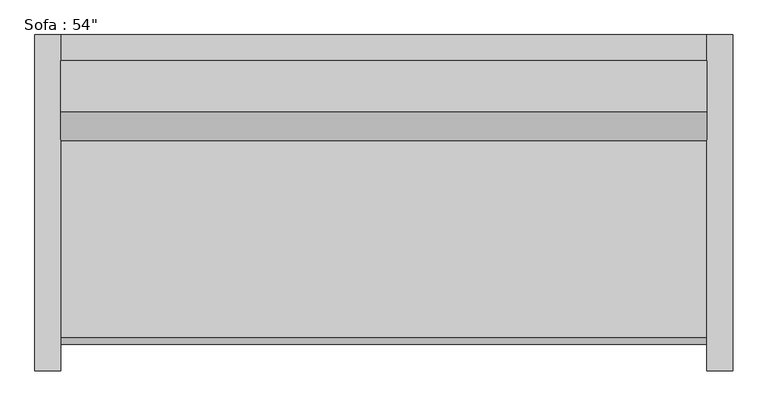
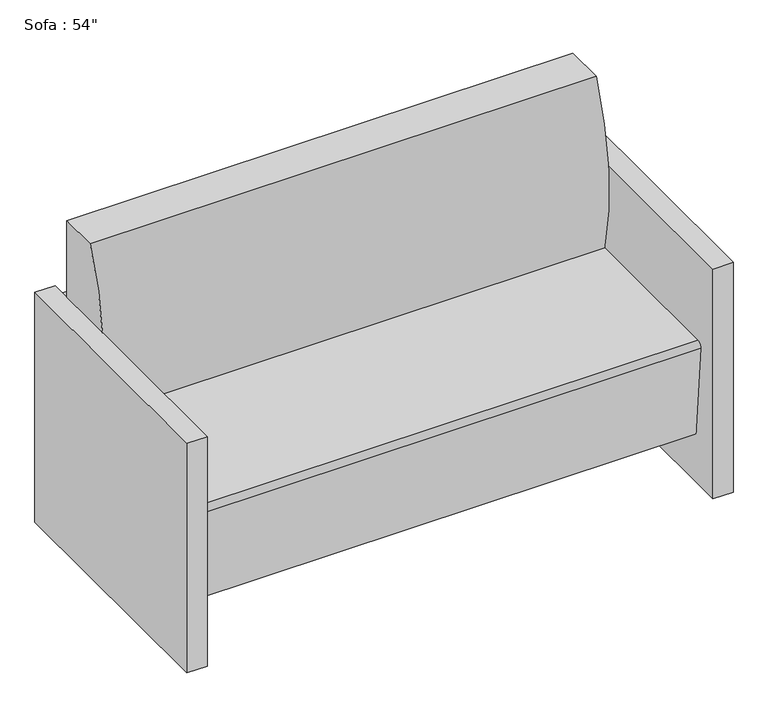
"""IFC4 building model written with IfcOpenShell, lengths in millimetres: furniture geometry."""

import ifcopenshell
import ifcopenshell.guid

model = None  # the IFC model being written
_history = None  # IfcOwnerHistory: only IFC2X3 demands one
_inside = {}  # id of a spatial element -> (the spatial element, [elements in it])
_under = {}  # id of a project, library or spatial element -> (it, [spatial elements below it])
_declared = {}  # id of a project -> (the project, [libraries it declares])
_typed = {}  # id of a type object -> (the type object, [elements of that type])
_made_of = {}  # id of a material, layer set ... -> (it, [elements and type objects made of it])


def new_model(schema):
    """Start an empty IFC model of exactly this schema.

    Asked for "IFC4X3", IfcOpenShell would pick the latest addendum, in which some entities
    have other attributes; the version numbers below select the first issue.
    IFC2X3 requires an IfcOwnerHistory on every rooted entity: one is made here for all.
    """
    global model, _history
    if schema == "IFC4X3":
        model = ifcopenshell.file(schema_version=(4, 3, 0, 0))
    else:
        model = ifcopenshell.file(schema=schema)
    _inside.clear()
    _under.clear()
    _declared.clear()
    _typed.clear()
    _made_of.clear()
    _history = None
    if model.schema == "IFC2X3":
        org = make("IfcOrganization", Name="unknown")
        user = make(
            "IfcPersonAndOrganization",
            ThePerson=make("IfcPerson", FamilyName="unknown"),
            TheOrganization=org,
        )
        app = make(
            "IfcApplication",
            ApplicationDeveloper=org,
            Version="unknown",
            ApplicationFullName="unknown",
            ApplicationIdentifier="unknown",
        )
        _history = make(
            "IfcOwnerHistory",
            OwningUser=user,
            OwningApplication=app,
            ChangeAction="ADDED",
            CreationDate=0,
        )
    return model


def make(cls, **values):
    """One entity of the class cls with the attributes given. An attribute that is None is left unset."""
    return model.create_entity(
        cls, **{name: value for name, value in values.items() if value is not None}
    )


def rooted(cls, **values):
    """An entity with a GlobalId (a new one), such as an element, a storey or a relation."""
    return make(cls, GlobalId=ifcopenshell.guid.new(), OwnerHistory=_history, **values)


def si_unit(unit_type, name, prefix=None):
    """IfcSIUnit, for example si_unit("LENGTHUNIT", "METRE", prefix="MILLI")."""
    return make("IfcSIUnit", UnitType=unit_type, Prefix=prefix, Name=name)


def assignment(units):
    """IfcUnitAssignment: the units of a project."""
    return None if units is None else make("IfcUnitAssignment", Units=units)


def point(xyz):
    """IfcCartesianPoint."""
    return None if xyz is None else make("IfcCartesianPoint", Coordinates=xyz)


def direction(xyz):
    """IfcDirection."""
    return None if xyz is None else make("IfcDirection", DirectionRatios=xyz)


def frame(location, z_axis=None, x_axis=None):
    """IfcAxis2Placement3D, a coordinate frame: its origin and axes. An axis left out is left unset."""
    return make(
        "IfcAxis2Placement3D",
        Location=point(location),
        Axis=direction(z_axis),
        RefDirection=direction(x_axis),
    )


def frame_2d(location, x_axis=None):
    """IfcAxis2Placement2D, a coordinate frame in the plane: its origin and x axis."""
    return make(
        "IfcAxis2Placement2D", Location=point(location), RefDirection=direction(x_axis)
    )


def origin():
    """The frame at (0, 0, 0) with its axes left unset."""
    return frame((0.0, 0.0, 0.0))


def origin_with_axes():
    """The frame at (0, 0, 0) with the z axis (0, 0, 1) and the x axis (1, 0, 0) written out."""
    return frame((0.0, 0.0, 0.0), z_axis=(0.0, 0.0, 1.0), x_axis=(1.0, 0.0, 0.0))


def place(relative_to, where):
    """IfcLocalPlacement: puts the frame where relative to a parent placement (None: the world)."""
    return make(
        "IfcLocalPlacement", PlacementRelTo=relative_to, RelativePlacement=where
    )


def context(
    kind, dimensions, precision=None, world=None, true_north=None, identifier=None
):
    """IfcGeometricRepresentationContext, for example the 3D "Model" context."""
    return make(
        "IfcGeometricRepresentationContext",
        ContextIdentifier=identifier,
        ContextType=kind,
        CoordinateSpaceDimension=dimensions,
        Precision=precision,
        WorldCoordinateSystem=world,
        TrueNorth=true_north,
    )


def project(units=None, contexts=None):
    """IfcProject with its units and contexts."""
    return rooted(
        "IfcProject",
        Name="project",
        RepresentationContexts=contexts,
        UnitsInContext=assignment(units),
    )


def spatial(cls, under=None, at=None, **own):
    """A site, building, storey or space (cls), placed at a placement, below another one or the project."""
    s = rooted(cls, ObjectPlacement=at, **own)
    if under is not None:
        _under.setdefault(under.id(), (under, []))[1].append(s)
    return s


def polyline(points):
    """IfcPolyline through the points."""
    return make("IfcPolyline", Points=[point(p) for p in points])


def circle_curve(where, radius):
    """IfcCircle in the frame where."""
    return make("IfcCircle", Position=where, Radius=radius)


def trimmed(basis, trim1, trim2, sense, master):
    """IfcTrimmedCurve: the piece of a basis curve between two trims."""
    return make(
        "IfcTrimmedCurve",
        BasisCurve=basis,
        Trim1=trim1,
        Trim2=trim2,
        SenseAgreement=sense,
        MasterRepresentation=master,
    )


def segment(curve, same_sense, transition):
    """IfcCompositeCurveSegment."""
    return make(
        "IfcCompositeCurveSegment",
        Transition=transition,
        SameSense=same_sense,
        ParentCurve=curve,
    )


def composite_curve(segments, self_intersect=None):
    """IfcCompositeCurve: segments joined end to end."""
    return make("IfcCompositeCurve", Segments=segments, SelfIntersect=self_intersect)


def outline(outer, holes=None, kind="AREA"):
    """IfcArbitraryClosedProfileDef: a profile drawn as a closed curve; with holes, ...WithVoids."""
    if holes is None:
        return make("IfcArbitraryClosedProfileDef", ProfileType=kind, OuterCurve=outer)
    return make(
        "IfcArbitraryProfileDefWithVoids",
        ProfileType=kind,
        OuterCurve=outer,
        InnerCurves=holes,
    )


def extrude(swept, where, along, depth):
    """IfcExtrudedAreaSolid: the profile swept, set in the frame where, extruded along a direction by depth."""
    return make(
        "IfcExtrudedAreaSolid",
        SweptArea=swept,
        Position=where,
        ExtrudedDirection=direction(along),
        Depth=depth,
    )


def shape(context_of_items, identifier, shape_type, items):
    """IfcShapeRepresentation: the items that make up one representation, for example the "Body"."""
    return make(
        "IfcShapeRepresentation",
        ContextOfItems=context_of_items,
        RepresentationIdentifier=identifier,
        RepresentationType=shape_type,
        Items=items,
    )


def source(mapping_origin, context_of_items, identifier, shape_type, items):
    """IfcRepresentationMap: a shape defined once, which mapped items show again and again."""
    return make(
        "IfcRepresentationMap",
        MappingOrigin=mapping_origin,
        MappedRepresentation=shape(context_of_items, identifier, shape_type, items),
    )


def transform(
    local_origin,
    x_axis=None,
    y_axis=None,
    z_axis=None,
    scale=None,
    scale2=None,
    scale3=None,
    uniform=True,
):
    """IfcCartesianTransformationOperator3D, or its non-uniform kind. x_axis, y_axis, z_axis: its Axis1, 2, 3."""
    if uniform:
        return make(
            "IfcCartesianTransformationOperator3D",
            Axis1=direction(x_axis),
            Axis2=direction(y_axis),
            LocalOrigin=point(local_origin),
            Scale=scale,
            Axis3=direction(z_axis),
        )
    return make(
        "IfcCartesianTransformationOperator3DnonUniform",
        Axis1=direction(x_axis),
        Axis2=direction(y_axis),
        LocalOrigin=point(local_origin),
        Scale=scale,
        Axis3=direction(z_axis),
        Scale2=scale2,
        Scale3=scale3,
    )


def mapped(mapping_source, mapping_target):
    """IfcMappedItem: shows the shape of a source again, moved by a transform."""
    return make(
        "IfcMappedItem", MappingSource=mapping_source, MappingTarget=mapping_target
    )


def made_of(thing, what):
    """Note that an element or type object is made of a material, layer set ...; save() writes the relation."""
    if what is not None:
        _made_of.setdefault(what.id(), (what, []))[1].append(thing)
    return thing


def element(
    cls,
    number,
    at=None,
    inside=None,
    cuts=None,
    type_object=None,
    material=None,
    context=None,
    identifier="Body",
    shape_type=None,
    held_by="IfcProductDefinitionShape",
    body=None,
    shapes=None,
    **own,
):
    """One element of the class cls, such as IfcWall. Its Tag is "e" and its number.

    at: its placement. inside: the storey or other place that contains it. cuts: it is an
    opening in that element (IfcRelVoidsElement). A single representation is given by context,
    identifier, shape_type and body (its items); several are given by shapes. held_by: the class
    of the entity that holds the representations. save() writes the other relations.
    """
    e = rooted(cls, Tag="e%d" % number, ObjectPlacement=at, **own)
    if body is not None:
        shapes = [shape(context, identifier, shape_type, body)]
    if shapes is not None:
        e.Representation = make(held_by, Representations=shapes)
    if inside is not None:
        _inside.setdefault(inside.id(), (inside, []))[1].append(e)
    if cuts is not None:
        rooted(
            "IfcRelVoidsElement", RelatingBuildingElement=cuts, RelatedOpeningElement=e
        )
    if type_object is not None:
        _typed.setdefault(type_object.id(), (type_object, []))[1].append(e)
    return made_of(e, material)


def aggregate(whole, parts):
    """IfcRelAggregates: a whole, such as a stair, and the parts it consists of."""
    return rooted("IfcRelAggregates", RelatingObject=whole, RelatedObjects=parts)


def save(model, path):
    """Write the relations noted so far, then the file.

    IfcRelAggregates (storeys below a building ...), IfcRelContainedInSpatialStructure (elements
    in a storey), IfcRelDefinesByType, IfcRelAssociatesMaterial and IfcRelDeclares: one each for
    every whole, place, type object, material and project.
    """
    for whole, parts in _under.values():
        aggregate(whole, parts)
    for where, things in _inside.values():
        rooted(
            "IfcRelContainedInSpatialStructure",
            RelatedElements=things,
            RelatingStructure=where,
        )
    for kind, things in _typed.values():
        rooted("IfcRelDefinesByType", RelatedObjects=things, RelatingType=kind)
    for what, things in _made_of.values():
        rooted("IfcRelAssociatesMaterial", RelatedObjects=things, RelatingMaterial=what)
    for by, libraries in _declared.values():
        rooted("IfcRelDeclares", RelatingContext=by, RelatedDefinitions=libraries)
    model.write(path)


def furniture_22419f35(model_context):
    return source(origin(), model_context, "Body", "SweptSolid", [
        extrude(outline(polyline([(-564.6295082, 425.5540984), (-564.6295082, 476.3540984), (705.3704918, 476.3540984), (705.3704918, 425.5540984), (-564.6295082, 425.5540984)])), frame((0.0, 0.0, 457.2), z_axis=(0.0, 0.0, 1.0), x_axis=(1.0, 0.0, 0.0)), (0.0, 0.0, 1.0), 127.0),
        extrude(outline(polyline([(-564.6295082, 425.5540984), (-564.6295082, 476.3540984), (705.3704918, 476.3540984), (705.3704918, 425.5540984), (-564.6295082, 425.5540984)])), frame((0.0, 0.0, 266.7), z_axis=(0.0, 0.0, 1.0), x_axis=(1.0, 0.0, 0.0)), (0.0, 0.0, 1.0), 127.0),
        extrude(outline(polyline([(-564.6295082, 425.5540984), (-564.6295082, 476.3540984), (705.3704918, 476.3540984), (705.3704918, 425.5540984), (-564.6295082, 425.5540984)])), frame((0.0, 0.0, 76.2), z_axis=(0.0, 0.0, 1.0), x_axis=(1.0, 0.0, 0.0)), (0.0, 0.0, 1.0), 127.0),
        extrude(outline(composite_curve([segment(trimmed(circle_curve(frame_2d((926.517198, 542.5300036)), 660.4), [point((286.1764935, 381.0))], [point((323.9540984, 812.8))], False, "CARTESIAN"), True, "CONTINUOUS"), segment(polyline([(323.9540984, 812.8), (425.5540984, 812.8), (425.5540984, 127.9665467), (-111.108343, 127.9665467), (-132.0379563, 367.1931221)]), True, "CONTINUOUS"), segment(trimmed(circle_curve(frame_2d((-119.3862837, 368.3)), 12.7), [point((-132.0379563, 367.1931221))], [point((-119.3862837, 381.0))], False, "CARTESIAN"), True, "CONTINUOUS"), segment(polyline([(-119.3862837, 381.0), (286.1764935, 381.0)]), True, "CONTINUOUS")], self_intersect=False)), frame((-564.6295082, 0.0, 0.0), z_axis=(1.0, 0.0, 0.0), x_axis=(0.0, 1.0, 0.0)), (0.0, 0.0, 1.0), 1270.0),
        extrude(outline(polyline([(-615.4295082, 476.3540984), (-564.6295082, 476.3540984), (-564.6295082, -184.0459016), (-615.4295082, -184.0459016), (-615.4295082, 476.3540984)])), origin_with_axes(), (0.0, 0.0, 1.0), 609.6),
        extrude(outline(polyline([(756.1704918, 476.3540984), (756.1704918, -184.0459016), (705.3704918, -184.0459016), (705.3704918, 476.3540984), (756.1704918, 476.3540984)])), origin_with_axes(), (0.0, 0.0, 1.0), 609.6),
    ])


if __name__ == "__main__":
    model = new_model("IFC4")
    model_context = context("Model", 3, world=origin())
    ifc_project = project(units=[si_unit("LENGTHUNIT", "METRE", prefix="MILLI")], contexts=[model_context])
    site = spatial("IfcSite", under=ifc_project)
    building = spatial("IfcBuilding", under=site)
    placement = place(None, origin())
    furniture_shape = furniture_22419f35(model_context)
    element("IfcFurniture", 1, ObjectType="Sofa : 54\"", at=placement, inside=building, context=model_context, shape_type="MappedRepresentation", body=[
        mapped(furniture_shape, transform((0.0, 0.0, 0.0), x_axis=(1.0, 0.0, 0.0), y_axis=(0.0, 1.0, 0.0), z_axis=(0.0, 0.0, 1.0))),
    ])
    save(model, "model.ifc")

# Revit data of these elements
# Type "Sofa : 54\""
#   Assembly Code = "E2020200"
#   Width = 4' - 6"
#   Seat Material = none
#   Frame Material = none
#   Default Elevation = 0
# Element 1 (IfcFurniture, "Sofa : 54\"")
#   Materials on its faces: "Cherry"
# Materials
#   "Cherry": class "Wood", colour RGB 233 182 144, transparency 0, Description = "Prunus Serotina", Cost = 0
